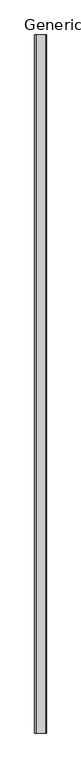
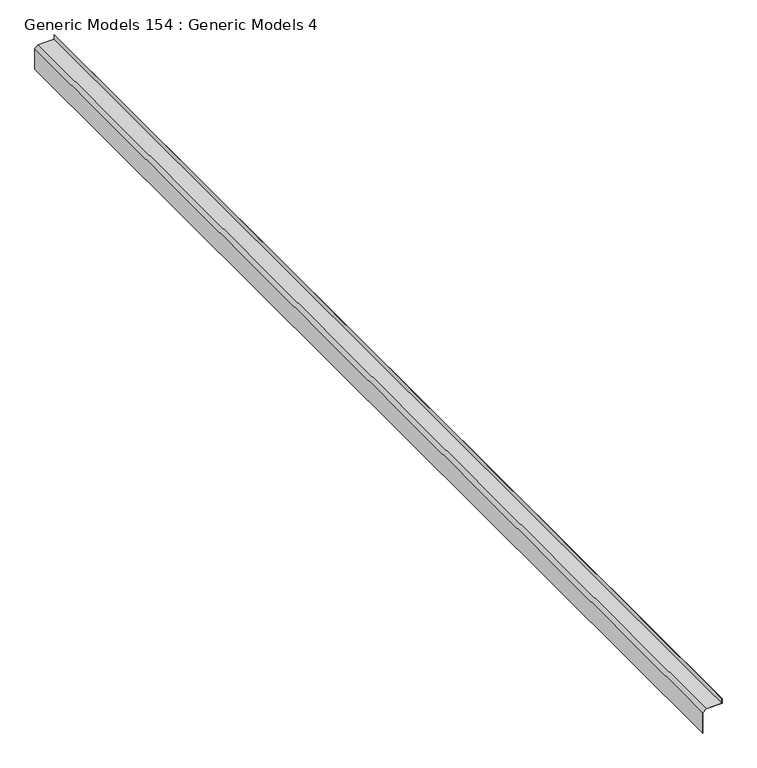
"""IFC4 building model written with IfcOpenShell, lengths in millimetres: proxy geometry, Generic Models 154 : Generic Models 4."""

from ifc_helpers import new_model, si_unit, frame, origin, place, context, project, spatial, polyline, outline, extrude, source, transform, mapped, element, save


def generic_models_154_generic_models_4_103a7c27(model_context):
    return source(origin(), model_context, "Body", "SweptSolid", [
        extrude(outline(polyline([(123262.4087349, -6500.9338375), (123294.9524849, -6500.9338375), (123294.9524849, -6501.7275875), (123263.2024849, -6501.7275875), (123263.2024849, -6610.1742668), (123241.0806267, -6632.2961251), (123094.7018446, -6632.2961251), (123094.7018446, -6631.5023751), (123240.7518446, -6631.5023751), (123262.4087349, -6609.8454848), (123262.4087349, -6500.9338375)])), frame((0.0, -5493.3230338, 0.0), z_axis=(0.0, 1.0, 0.0), x_axis=(0.0, 0.0, 1.0)), (0.0, 0.0, 1.0), 7886.7),
    ])


if __name__ == "__main__":
    model = new_model("IFC4")
    model_context = context("Model", 3, world=origin())
    ifc_project = project(units=[si_unit("LENGTHUNIT", "METRE", prefix="MILLI")], contexts=[model_context])
    site = spatial("IfcSite", under=ifc_project)
    building = spatial("IfcBuilding", under=site)
    placement = place(None, origin())
    generic_models_154_generic_models_4_shape = generic_models_154_generic_models_4_103a7c27(model_context)
    element("IfcBuildingElementProxy", 1, Name="Generic Models 154 : Generic Models 4", ObjectType="Generic Models 154 : Generic Models 4", at=placement, inside=building, context=model_context, shape_type="MappedRepresentation", body=[
        mapped(generic_models_154_generic_models_4_shape, transform((0.0, 0.0, 0.0), x_axis=(1.0, 0.0, 0.0), y_axis=(0.0, 1.0, 0.0), z_axis=(0.0, 0.0, 1.0))),
    ])
    save(model, "model.ifc")

# Revit data of these elements
# Element 1 (IfcBuildingElementProxy, "Generic Models 154 : Generic Models 4")
#   Materials on its faces: "_16 GA. COPPER BRAKE METAL FLASHING W/ END DAMS"
# Materials
#   "_16 GA. COPPER BRAKE METAL FLASHING W/ END DAMS": class "Generic", colour RGB 175 175 175, transparency 0, Cost = 0
